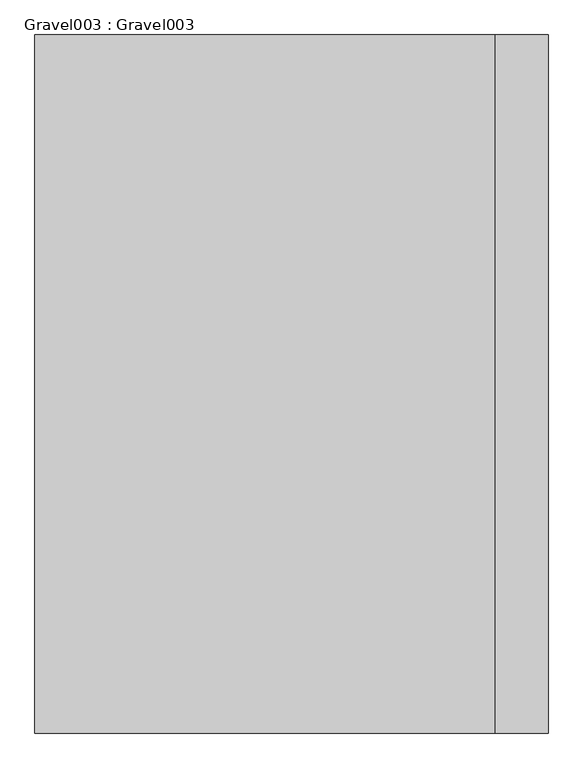
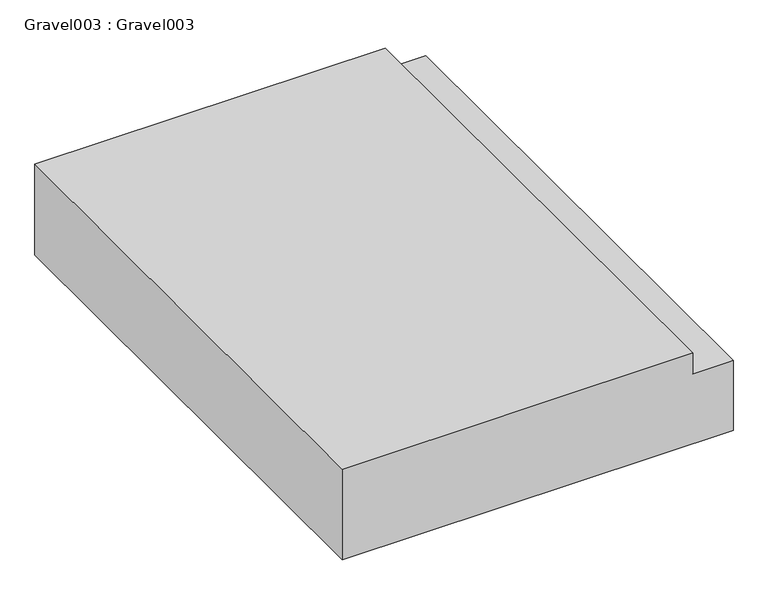
"""IFC4 building model written with IfcOpenShell, lengths in millimetres: proxy geometry, Gravel003 : Gravel003."""

from ifc_helpers import new_model, si_unit, frame, origin, place, context, project, spatial, polyline, outline, extrude, source, transform, mapped, element, save


def gravel003_gravel003_56ee6a12(model_context):
    return source(origin(), model_context, "Body", "SweptSolid", [
        extrude(outline(polyline([(32036.6025286, -10098.4737014), (32314.8961275, -10098.4737014), (32314.8961275, -10250.8737014), (32397.0602473, -10250.8737014), (32397.0602473, -11568.4300809), (32036.6025286, -11568.4300809), (32036.6025286, -10098.4737014)])), frame((0.0, 7982.1531721, 0.0), z_axis=(0.0, 1.0, 0.0), x_axis=(0.0, 0.0, 1.0)), (0.0, 0.0, 1.0), 2000.0),
    ])


if __name__ == "__main__":
    model = new_model("IFC4")
    model_context = context("Model", 3, world=origin())
    ifc_project = project(units=[si_unit("LENGTHUNIT", "METRE", prefix="MILLI")], contexts=[model_context])
    site = spatial("IfcSite", under=ifc_project)
    building = spatial("IfcBuilding", under=site)
    placement = place(None, origin())
    gravel003_gravel003_shape = gravel003_gravel003_56ee6a12(model_context)
    element("IfcBuildingElementProxy", 1, Name="Gravel003 : Gravel003", ObjectType="Gravel003 : Gravel003", at=placement, inside=building, context=model_context, shape_type="MappedRepresentation", body=[
        mapped(gravel003_gravel003_shape, transform((0.0, 0.0, 0.0), x_axis=(1.0, 0.0, 0.0), y_axis=(0.0, 1.0, 0.0), z_axis=(0.0, 0.0, 1.0))),
    ])
    save(model, "model.ifc")

# Revit data of these elements
# Type "Gravel003 : Gravel003"
#   NameOverride = "Gravel003"
# Element 1 (IfcBuildingElementProxy, "Gravel003 : Gravel003")
#   Materials on its faces: "4\" MIN. CRUSHED GRAVEL (NO FINES)"
# Materials
#   "4\" MIN. CRUSHED GRAVEL (NO FINES)": class "Unassigned", colour RGB 145 162 188, transparency 0, Cost = 0
